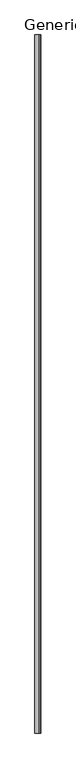
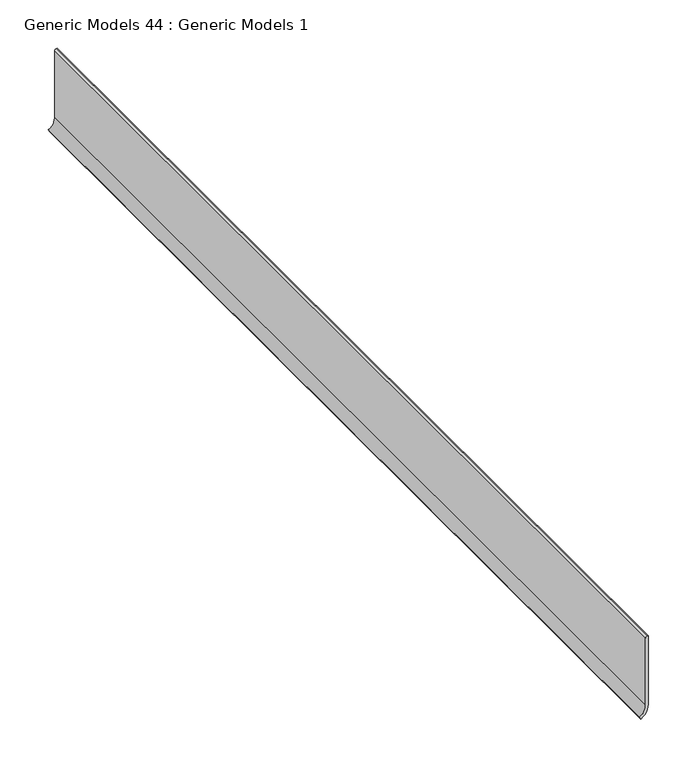
"""IFC4 building model written with IfcOpenShell, lengths in millimetres: proxy geometry, Generic Models 44 : Generic Models 1."""

from ifc_helpers import new_model, si_unit, point, frame, frame_2d, origin, place, context, project, spatial, polyline, circle_curve, trimmed, segment, composite_curve, outline, extrude, source, transform, mapped, element, save


def generic_models_44_generic_models_1_f536fb9f(model_context):
    return source(origin(), model_context, "Body", "SweptSolid", [
        extrude(outline(composite_curve([segment(polyline([(73.749588, 50688.3189813), (73.749588, 50687.2307831)]), True, "CONTINUOUS"), segment(trimmed(circle_curve(frame_2d((71.6627862, 50687.2307831)), 2.0868018), [point((73.749588, 50687.2307831))], [point((71.6627862, 50685.1439813))], False, "CARTESIAN"), True, "CONTINUOUS"), segment(polyline([(71.6627862, 50685.1439813), (-12.4007813, 50685.1439813)]), True, "CONTINUOUS"), segment(trimmed(circle_curve(frame_2d((-12.4007813, 50670.4792845)), 14.6646968), [point((-12.4007813, 50685.1439813))], [point((-25.1007813, 50677.8116329))], True, "CARTESIAN"), True, "CONTINUOUS"), segment(polyline([(-25.1007813, 50677.8116329), (-27.850412, 50679.3991329)]), True, "CONTINUOUS"), segment(trimmed(circle_curve(frame_2d((-12.4007813, 50670.4792845)), 17.8396968), [point((-27.850412, 50679.3991329))], [point((-12.4007813, 50688.3189813))], False, "CARTESIAN"), True, "CONTINUOUS"), segment(polyline([(-12.4007813, 50688.3189813), (73.749588, 50688.3189813)]), True, "CONTINUOUS")], self_intersect=False)), frame((0.0, 0.0, 0.0), z_axis=(0.0, 1.0, 0.0), x_axis=(0.0, 0.0, 1.0)), (0.0, 0.0, 1.0), 1219.2),
    ])


if __name__ == "__main__":
    model = new_model("IFC4")
    model_context = context("Model", 3, world=origin())
    ifc_project = project(units=[si_unit("LENGTHUNIT", "METRE", prefix="MILLI")], contexts=[model_context])
    site = spatial("IfcSite", under=ifc_project)
    building = spatial("IfcBuilding", under=site)
    placement = place(None, origin())
    generic_models_44_generic_models_1_shape = generic_models_44_generic_models_1_f536fb9f(model_context)
    element("IfcBuildingElementProxy", 1, Name="Generic Models 44 : Generic Models 1", ObjectType="Generic Models 44 : Generic Models 1", at=placement, inside=building, context=model_context, shape_type="MappedRepresentation", body=[
        mapped(generic_models_44_generic_models_1_shape, transform((0.0, 0.0, 0.0), x_axis=(1.0, 0.0, 0.0), y_axis=(0.0, 1.0, 0.0), z_axis=(0.0, 0.0, 1.0))),
    ])
    save(model, "model.ifc")

# Revit data of these elements
# Element 1 (IfcBuildingElementProxy, "Generic Models 44 : Generic Models 1")
#   Materials on its faces: "BASE AS SCHEDULED"
# Materials
#   "BASE AS SCHEDULED": class "Generic", colour RGB 120 120 120, transparency 0, Cost = 0
